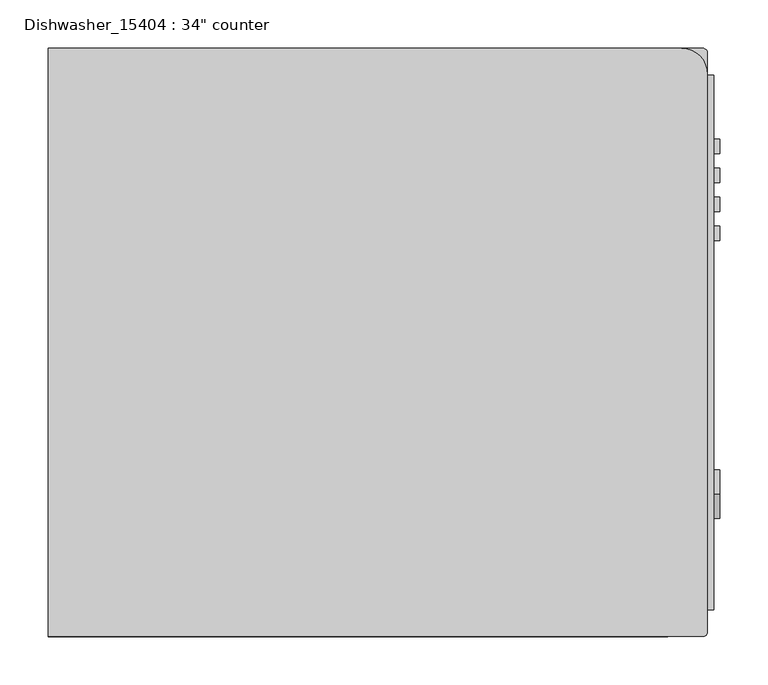
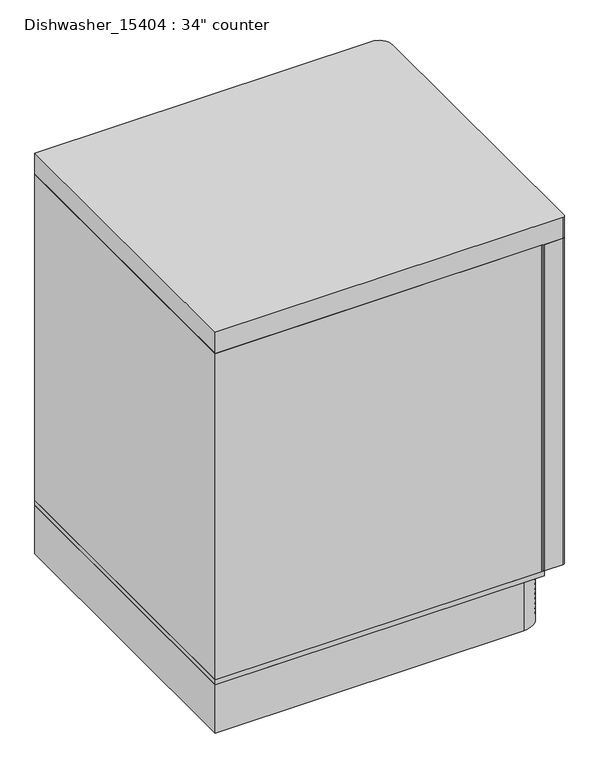
"""IFC4 building model written with IfcOpenShell, lengths in millimetres: proxy geometry."""

from ifc_helpers import new_model, si_unit, point, frame, frame_2d, origin, place, context, project, spatial, polyline, circle_curve, trimmed, segment, composite_curve, outline, extrude, source, transform, mapped, element, save
from ifc_brep_helpers import plane_surface, cylinder_surface, advanced_brep


def proxy_e1c3c540(model_context):
    return source(origin(), model_context, "Body", "SolidModel", [
        extrude(outline(composite_curve([segment(trimmed(circle_curve(frame_2d((147.53066, 741.5840355)), 25.0), [point((147.53066, 716.5840355))], [point((147.53066, 766.5840355))], False, "CARTESIAN"), True, "CONTINUOUS"), segment(trimmed(circle_curve(frame_2d((147.53066, 741.5840355)), 25.0), [point((147.53066, 766.5840355))], [point((147.53066, 716.5840355))], False, "CARTESIAN"), True, "CONTINUOUS")], self_intersect=False)), frame((688.975, 0.0, 0.0), z_axis=(1.0, 0.0, 0.0), x_axis=(0.0, 1.0, 0.0)), (0.0, 0.0, 1.0), 6.35),
        extrude(outline(polyline([(688.975, 410.2108979), (688.975, 425.2108979), (695.325, 425.2108979), (695.325, 410.2108979), (688.975, 410.2108979)])), frame((0.0, 0.0, 745.4030607), z_axis=(0.0, 0.0, 1.0), x_axis=(1.0, 0.0, 0.0)), (0.0, 0.0, 1.0), 15.0),
        extrude(outline(polyline([(688.975, 440.2108979), (688.975, 455.2108979), (695.325, 455.2108979), (695.325, 440.2108979), (688.975, 440.2108979)])), frame((0.0, 0.0, 745.4030607), z_axis=(0.0, 0.0, 1.0), x_axis=(1.0, 0.0, 0.0)), (0.0, 0.0, 1.0), 15.0),
        extrude(outline(polyline([(688.975, 470.2108979), (688.975, 485.2108979), (695.325, 485.2108979), (695.325, 470.2108979), (688.975, 470.2108979)])), frame((0.0, 0.0, 745.4030607), z_axis=(0.0, 0.0, 1.0), x_axis=(1.0, 0.0, 0.0)), (0.0, 0.0, 1.0), 15.0),
        extrude(outline(polyline([(688.975, 500.2108979), (688.975, 515.2108979), (695.325, 515.2108979), (695.325, 500.2108979), (688.975, 500.2108979)])), frame((0.0, 0.0, 745.4030607), z_axis=(0.0, 0.0, 1.0), x_axis=(1.0, 0.0, 0.0)), (0.0, 0.0, 1.0), 15.0),
        extrude(outline(composite_curve([segment(polyline([(512.7209143, 694.5980964), (96.8794309, 694.5980964)]), True, "CONTINUOUS"), segment(trimmed(circle_curve(frame_2d((96.8794309, 729.5980964)), 35.0), [point((96.8794309, 694.5980964))], [point((66.2677412, 712.6297597))], False, "CARTESIAN"), True, "CONTINUOUS"), segment(polyline([(66.2677412, 712.6297597), (27.7608134, 782.0980964), (581.8395319, 782.0980964), (543.3326041, 712.6297597)]), True, "CONTINUOUS"), segment(trimmed(circle_curve(frame_2d((512.7209143, 729.5980964)), 35.0), [point((543.3326041, 712.6297597))], [point((512.7209143, 694.5980964))], False, "CARTESIAN"), True, "CONTINUOUS")], self_intersect=False)), frame((638.175, 0.0, 0.0), z_axis=(1.0, 0.0, 0.0), x_axis=(0.0, 1.0, 0.0)), (0.0, 0.0, 1.0), 50.8),
        extrude(outline(composite_curve([segment(polyline([(0.0, 609.6), (636.35, 609.6)]), True, "CONTINUOUS"), segment(trimmed(circle_curve(frame_2d((636.35, 604.6)), 5.0), [point((636.35, 609.6))], [point((641.35, 604.6))], False, "CARTESIAN"), True, "CONTINUOUS"), segment(polyline([(641.35, 604.6), (641.35, 5.0003453)]), True, "CONTINUOUS"), segment(trimmed(circle_curve(frame_2d((636.35, 5.0003453)), 5.0), [point((641.35, 5.0003453))], [point((636.35, 0.0003453))], False, "CARTESIAN"), True, "CONTINUOUS"), segment(polyline([(636.35, 0.0003453), (0.0, 0.0003453), (0.0, 609.6)]), True, "CONTINUOUS")], self_intersect=False)), frame((0.0, 0.0, 110.0), z_axis=(0.0, 0.0, 1.0), x_axis=(1.0, 0.0, 0.0)), (0.0, 0.0, 1.0), 672.0980964),
        extrude(outline(composite_curve([segment(polyline([(0.0, 609.6), (655.4, 609.6)]), True, "CONTINUOUS"), segment(trimmed(circle_curve(frame_2d((655.4, 582.375)), 27.225), [point((655.4, 609.6))], [point((682.625, 582.375))], False, "CARTESIAN"), True, "CONTINUOUS"), segment(polyline([(682.625, 582.375), (682.625, 5.0)]), True, "CONTINUOUS"), segment(trimmed(circle_curve(frame_2d((677.625, 5.0)), 5.0), [point((682.625, 5.0))], [point((677.625, 0.0))], False, "CARTESIAN"), True, "CONTINUOUS"), segment(polyline([(677.625, 0.0), (0.0, 0.0), (0.0, 609.6)]), True, "CONTINUOUS")], self_intersect=False)), frame((0.0, 0.0, 782.0980964), z_axis=(0.0, 0.0, 1.0), x_axis=(1.0, 0.0, 0.0)), (0.0, 0.0, 1.0), 43.4019036),
        extrude(outline(composite_curve([segment(polyline([(641.35, 609.6), (677.625, 609.6)]), True, "CONTINUOUS"), segment(trimmed(circle_curve(frame_2d((677.625, 604.6)), 5.0), [point((677.625, 609.6))], [point((682.625, 604.6))], False, "CARTESIAN"), True, "CONTINUOUS"), segment(polyline([(682.625, 604.6), (682.625, 5.0)]), True, "CONTINUOUS"), segment(trimmed(circle_curve(frame_2d((677.625, 5.0)), 5.0), [point((682.625, 5.0))], [point((677.625, 0.0))], False, "CARTESIAN"), True, "CONTINUOUS"), segment(polyline([(677.625, 0.0), (641.35, 0.0), (641.35, 609.6)]), True, "CONTINUOUS")], self_intersect=False)), frame((0.0, 0.0, 110.0), z_axis=(0.0, 0.0, 1.0), x_axis=(1.0, 0.0, 0.0)), (0.0, 0.0, 1.0), 672.0980964),
        extrude(outline(polyline([(0.0, 609.6), (641.35, 609.6), (641.35, 0.0), (0.0, 0.0), (0.0, 609.6)])), frame((0.0, 0.0, 100.0), z_axis=(0.0, 0.0, 1.0), x_axis=(1.0, 0.0, 0.0)), (0.0, 0.0, 1.0), 10.0),
        advanced_brep(
        [(0.0, 609.6, 100.0), (0.0, 0.0, 100.0), (601.35, 0.0, 100.0), (641.35, 40.0, 100.0), (641.35, 569.6, 100.0), (601.35, 609.6, 100.0), (0.0, 609.6, 0.0), (601.35, 609.6, 0.0), (641.35, 569.6, 0.0), (641.35, 40.0, 0.0), (601.35, 0.0, 0.0), (0.0, 0.0, 0.0), (641.35, 40.0, 16.3757772), (628.65, 10.7645763, 16.3757772), (628.65, 10.7645763, 21.3757772), (641.35, 40.0, 21.3757772), (641.35, 40.0, 26.2238547), (628.65, 10.7645763, 26.2238547), (628.65, 10.7645763, 31.2238547), (641.35, 40.0, 31.2238547), (641.35, 40.0, 36.2238547), (628.65, 10.7645763, 36.2238547), (628.65, 10.7645763, 41.2238547), (641.35, 40.0, 41.2238547), (641.35, 40.0, 46.2238547), (628.65, 10.7645763, 46.2238547), (628.65, 10.7645763, 51.2238547), (641.35, 40.0, 51.2238547), (641.35, 40.0, 56.2238547), (628.65, 10.7645763, 56.2238547), (628.65, 10.7645763, 61.2238547), (641.35, 40.0, 61.2238547), (641.35, 40.0, 66.2238547), (628.65, 10.7645763, 66.2238547), (628.65, 10.7645763, 71.2238547), (641.35, 40.0, 71.2238547), (641.35, 40.0, 76.2238547), (628.65, 10.7645763, 76.2238547), (628.65, 10.7645763, 81.2238547), (641.35, 40.0, 81.2238547), (641.35, 40.0, 86.2238547), (628.65, 10.7645763, 86.2238547), (628.65, 10.7645763, 91.2238547), (641.35, 40.0, 91.2238547), (641.35, 569.6, 91.2238547), (641.35, 569.6, 16.3757772), (641.35, 569.6, 21.3757772), (641.35, 569.6, 26.2238547), (641.35, 569.6, 31.2238547), (641.35, 569.6, 36.2238547), (641.35, 569.6, 41.2238547), (641.35, 569.6, 46.2238547), (641.35, 569.6, 51.2238547), (641.35, 569.6, 56.2238547), (641.35, 569.6, 61.2238547), (641.35, 569.6, 66.2238547), (641.35, 569.6, 71.2238547), (641.35, 569.6, 76.2238547), (641.35, 569.6, 81.2238547), (641.35, 569.6, 86.2238547), (628.65, 598.8354237, 91.2238547), (628.65, 598.8354237, 86.2238547), (628.65, 598.8354237, 81.2238547), (628.65, 598.8354237, 76.2238547), (628.65, 598.8354237, 71.2238547), (628.65, 598.8354237, 66.2238547), (628.65, 598.8354237, 61.2238547), (628.65, 598.8354237, 56.2238547), (628.65, 598.8354237, 51.2238547), (628.65, 598.8354237, 46.2238547), (628.65, 598.8354237, 41.2238547), (628.65, 598.8354237, 36.2238547), (628.65, 598.8354237, 31.2238547), (628.65, 598.8354237, 26.2238547), (628.65, 598.8354237, 21.3757772), (628.65, 598.8354237, 16.3757772)],
        [
            (0, 1),
            (1, 2),
            (2, 3, circle_curve(frame((601.35, 40.0, 100.0), z_axis=(0.0, 0.0, 1.0), x_axis=(1.0, 0.0, 0.0)), 40.0)),
            (3, 4),
            (4, 5, circle_curve(frame((601.35, 569.6, 100.0), z_axis=(0.0, 0.0, 1.0), x_axis=(1.0, 0.0, 0.0)), 40.0)),
            (5, 0),
            (6, 7),
            (7, 8, circle_curve(frame((601.35, 569.6, 0.0), z_axis=(0.0, 0.0, -1.0), x_axis=(1.0, 0.0, 0.0)), 40.0)),
            (8, 9),
            (9, 10, circle_curve(frame((601.35, 40.0, 0.0), z_axis=(0.0, 0.0, -1.0), x_axis=(1.0, 0.0, 0.0)), 40.0)),
            (10, 11),
            (11, 6),
            (0, 6),
            (11, 1),
            (10, 2),
            (9, 12),
            (12, 13, circle_curve(frame((601.35, 40.0, 16.3757772), z_axis=(0.0, 0.0, -1.0), x_axis=(1.0, 0.0, 0.0)), 40.0)),
            (13, 14),
            (14, 15, circle_curve(frame((601.35, 40.0, 21.3757772), z_axis=(0.0, 0.0, 1.0), x_axis=(1.0, 0.0, 0.0)), 40.0)),
            (15, 16),
            (16, 17, circle_curve(frame((601.35, 40.0, 26.2238547), z_axis=(0.0, 0.0, -1.0), x_axis=(1.0, 0.0, 0.0)), 40.0)),
            (17, 18),
            (18, 19, circle_curve(frame((601.35, 40.0, 31.2238547), z_axis=(0.0, 0.0, 1.0), x_axis=(1.0, 0.0, 0.0)), 40.0)),
            (19, 20),
            (20, 21, circle_curve(frame((601.35, 40.0, 36.2238547), z_axis=(0.0, 0.0, -1.0), x_axis=(1.0, 0.0, 0.0)), 40.0)),
            (21, 22),
            (22, 23, circle_curve(frame((601.35, 40.0, 41.2238547), z_axis=(0.0, 0.0, 1.0), x_axis=(1.0, 0.0, 0.0)), 40.0)),
            (23, 24),
            (24, 25, circle_curve(frame((601.35, 40.0, 46.2238547), z_axis=(0.0, 0.0, -1.0), x_axis=(1.0, 0.0, 0.0)), 40.0)),
            (25, 26),
            (26, 27, circle_curve(frame((601.35, 40.0, 51.2238547), z_axis=(0.0, 0.0, 1.0), x_axis=(1.0, 0.0, 0.0)), 40.0)),
            (27, 28),
            (28, 29, circle_curve(frame((601.35, 40.0, 56.2238547), z_axis=(0.0, 0.0, -1.0), x_axis=(1.0, 0.0, 0.0)), 40.0)),
            (29, 30),
            (30, 31, circle_curve(frame((601.35, 40.0, 61.2238547), z_axis=(0.0, 0.0, 1.0), x_axis=(1.0, 0.0, 0.0)), 40.0)),
            (31, 32),
            (32, 33, circle_curve(frame((601.35, 40.0, 66.2238547), z_axis=(0.0, 0.0, -1.0), x_axis=(1.0, 0.0, 0.0)), 40.0)),
            (33, 34),
            (34, 35, circle_curve(frame((601.35, 40.0, 71.2238547), z_axis=(0.0, 0.0, 1.0), x_axis=(1.0, 0.0, 0.0)), 40.0)),
            (35, 36),
            (36, 37, circle_curve(frame((601.35, 40.0, 76.2238547), z_axis=(0.0, 0.0, -1.0), x_axis=(1.0, 0.0, 0.0)), 40.0)),
            (37, 38),
            (38, 39, circle_curve(frame((601.35, 40.0, 81.2238547), z_axis=(0.0, 0.0, 1.0), x_axis=(1.0, 0.0, 0.0)), 40.0)),
            (39, 40),
            (40, 41, circle_curve(frame((601.35, 40.0, 86.2238547), z_axis=(0.0, 0.0, -1.0), x_axis=(1.0, 0.0, 0.0)), 40.0)),
            (41, 42),
            (42, 43, circle_curve(frame((601.35, 40.0, 91.2238547), z_axis=(0.0, 0.0, 1.0), x_axis=(1.0, 0.0, 0.0)), 40.0)),
            (43, 3),
            (43, 44),
            (44, 4),
            (8, 45),
            (45, 12),
            (15, 46),
            (46, 47),
            (47, 16),
            (19, 48),
            (48, 49),
            (49, 20),
            (23, 50),
            (50, 51),
            (51, 24),
            (27, 52),
            (52, 53),
            (53, 28),
            (31, 54),
            (54, 55),
            (55, 32),
            (35, 56),
            (56, 57),
            (57, 36),
            (39, 58),
            (58, 59),
            (59, 40),
            (44, 60, circle_curve(frame((601.35, 569.6, 91.2238547), z_axis=(0.0, 0.0, 1.0), x_axis=(1.0, 0.0, 0.0)), 40.0)),
            (60, 61),
            (61, 59, circle_curve(frame((601.35, 569.6, 86.2238547), z_axis=(0.0, 0.0, -1.0), x_axis=(1.0, 0.0, 0.0)), 40.0)),
            (58, 62, circle_curve(frame((601.35, 569.6, 81.2238547), z_axis=(0.0, 0.0, 1.0), x_axis=(1.0, 0.0, 0.0)), 40.0)),
            (62, 63),
            (63, 57, circle_curve(frame((601.35, 569.6, 76.2238547), z_axis=(0.0, 0.0, -1.0), x_axis=(1.0, 0.0, 0.0)), 40.0)),
            (56, 64, circle_curve(frame((601.35, 569.6, 71.2238547), z_axis=(0.0, 0.0, 1.0), x_axis=(1.0, 0.0, 0.0)), 40.0)),
            (64, 65),
            (65, 55, circle_curve(frame((601.35, 569.6, 66.2238547), z_axis=(0.0, 0.0, -1.0), x_axis=(1.0, 0.0, 0.0)), 40.0)),
            (54, 66, circle_curve(frame((601.35, 569.6, 61.2238547), z_axis=(0.0, 0.0, 1.0), x_axis=(1.0, 0.0, 0.0)), 40.0)),
            (66, 67),
            (67, 53, circle_curve(frame((601.35, 569.6, 56.2238547), z_axis=(0.0, 0.0, -1.0), x_axis=(1.0, 0.0, 0.0)), 40.0)),
            (52, 68, circle_curve(frame((601.35, 569.6, 51.2238547), z_axis=(0.0, 0.0, 1.0), x_axis=(1.0, 0.0, 0.0)), 40.0)),
            (68, 69),
            (69, 51, circle_curve(frame((601.35, 569.6, 46.2238547), z_axis=(0.0, 0.0, -1.0), x_axis=(1.0, 0.0, 0.0)), 40.0)),
            (50, 70, circle_curve(frame((601.35, 569.6, 41.2238547), z_axis=(0.0, 0.0, 1.0), x_axis=(1.0, 0.0, 0.0)), 40.0)),
            (70, 71),
            (71, 49, circle_curve(frame((601.35, 569.6, 36.2238547), z_axis=(0.0, 0.0, -1.0), x_axis=(1.0, 0.0, 0.0)), 40.0)),
            (48, 72, circle_curve(frame((601.35, 569.6, 31.2238547), z_axis=(0.0, 0.0, 1.0), x_axis=(1.0, 0.0, 0.0)), 40.0)),
            (72, 73),
            (73, 47, circle_curve(frame((601.35, 569.6, 26.2238547), z_axis=(0.0, 0.0, -1.0), x_axis=(1.0, 0.0, 0.0)), 40.0)),
            (46, 74, circle_curve(frame((601.35, 569.6, 21.3757772), z_axis=(0.0, 0.0, 1.0), x_axis=(1.0, 0.0, 0.0)), 40.0)),
            (74, 75),
            (75, 45, circle_curve(frame((601.35, 569.6, 16.3757772), z_axis=(0.0, 0.0, -1.0), x_axis=(1.0, 0.0, 0.0)), 40.0)),
            (7, 5),
            (60, 42),
            (41, 61),
            (62, 38),
            (37, 63),
            (64, 34),
            (33, 65),
            (66, 30),
            (29, 67),
            (68, 26),
            (25, 69),
            (70, 22),
            (21, 71),
            (72, 18),
            (17, 73),
            (74, 14),
            (13, 75),
        ],
        [
            plane_surface(frame((0.0, 0.0, 100.0), z_axis=(0.0, 0.0, 1.0), x_axis=(0.0, -1.0, 0.0))),
            plane_surface(frame((0.0, 0.0, 0.0), z_axis=(0.0, 0.0, -1.0), x_axis=(0.0, 1.0, 0.0))),
            plane_surface(frame((0.0, 609.6, 100.0), z_axis=(-1.0, 0.0, 0.0), x_axis=(0.0, 0.0, -1.0))),
            plane_surface(frame((0.0, 0.0, 100.0), z_axis=(0.0, -1.0, 0.0), x_axis=(0.0, 0.0, -1.0))),
            cylinder_surface(frame((601.35, 40.0, 0.0), z_axis=(0.0, 0.0, 1.0), x_axis=(1.0, 0.0, 0.0)), 40.0),
            plane_surface(frame((641.35, 40.0, 100.0), z_axis=(1.0, 0.0, 0.0), x_axis=(0.0, 0.0, -1.0))),
            cylinder_surface(frame((601.35, 569.6, 0.0), z_axis=(0.0, 0.0, 1.0), x_axis=(1.0, 0.0, 0.0)), 40.0),
            plane_surface(frame((601.35, 609.6, 100.0), z_axis=(0.0, 1.0, 0.0), x_axis=(0.0, 0.0, -1.0))),
            plane_surface(frame((628.65, 0.0, 91.2238547), z_axis=(1.0, 0.0, 0.0), x_axis=(0.0, 1.0, 0.0))),
            plane_surface(frame((666.75, 609.6, 91.2238547), z_axis=(0.0, 0.0, -1.0), x_axis=(-1.0, 0.0, 0.0))),
            plane_surface(frame((666.75, 0.0, 86.2238547), z_axis=(0.0, 0.0, 1.0), x_axis=(-1.0, 0.0, 0.0))),
            plane_surface(frame((666.75, 609.6, 81.2238547), z_axis=(0.0, 0.0, -1.0), x_axis=(-1.0, 0.0, 0.0))),
            plane_surface(frame((666.75, 0.0, 76.2238547), z_axis=(0.0, 0.0, 1.0), x_axis=(-1.0, 0.0, 0.0))),
            plane_surface(frame((666.75, 609.6, 71.2238547), z_axis=(0.0, 0.0, -1.0), x_axis=(-1.0, 0.0, 0.0))),
            plane_surface(frame((666.75, 0.0, 66.2238547), z_axis=(0.0, 0.0, 1.0), x_axis=(-1.0, 0.0, 0.0))),
            plane_surface(frame((666.75, 609.6, 61.2238547), z_axis=(0.0, 0.0, -1.0), x_axis=(-1.0, 0.0, 0.0))),
            plane_surface(frame((666.75, 0.0, 56.2238547), z_axis=(0.0, 0.0, 1.0), x_axis=(-1.0, 0.0, 0.0))),
            plane_surface(frame((666.75, 609.6, 51.2238547), z_axis=(0.0, 0.0, -1.0), x_axis=(-1.0, 0.0, 0.0))),
            plane_surface(frame((666.75, 0.0, 46.2238547), z_axis=(0.0, 0.0, 1.0), x_axis=(-1.0, 0.0, 0.0))),
            plane_surface(frame((666.75, 609.6, 41.2238547), z_axis=(0.0, 0.0, -1.0), x_axis=(-1.0, 0.0, 0.0))),
            plane_surface(frame((666.75, 0.0, 36.2238547), z_axis=(0.0, 0.0, 1.0), x_axis=(-1.0, 0.0, 0.0))),
            plane_surface(frame((666.75, 609.6, 31.2238547), z_axis=(0.0, 0.0, -1.0), x_axis=(-1.0, 0.0, 0.0))),
            plane_surface(frame((666.75, 0.0, 26.2238547), z_axis=(0.0, 0.0, 1.0), x_axis=(-1.0, 0.0, 0.0))),
            plane_surface(frame((666.75, 609.6, 21.3757772), z_axis=(0.0, 0.0, -1.0), x_axis=(-1.0, 0.0, 0.0))),
            plane_surface(frame((666.75, 0.0, 16.3757772), z_axis=(0.0, 0.0, 1.0), x_axis=(-1.0, 0.0, 0.0))),
        ],
        [
            (0, [[1, 2, 3, 4, 5, 6]]),
            (1, [[7, 8, 9, 10, 11, 12]]),
            (2, [[-1, 13, -12, 14]]),
            (3, [[-2, -14, -11, 15]]),
            (4, [[-3, -15, -10, 16, 17, 18, 19, 20, 21, 22, 23, 24, 25, 26, 27, 28, 29, 30, 31, 32, 33, 34, 35, 36, 37, 38, 39, 40, 41, 42, 43, 44, 45, 46, 47, 48]]),
            (5, [[-4, -48, 49, 50]]),
            (5, [[-9, 51, 52, -16]]),
            (5, [[-20, 53, 54, 55]]),
            (5, [[-24, 56, 57, 58]]),
            (5, [[-28, 59, 60, 61]]),
            (5, [[-32, 62, 63, 64]]),
            (5, [[-36, 65, 66, 67]]),
            (5, [[-40, 68, 69, 70]]),
            (5, [[-44, 71, 72, 73]]),
            (6, [[-5, -50, 74, 75, 76, -72, 77, 78, 79, -69, 80, 81, 82, -66, 83, 84, 85, -63, 86, 87, 88, -60, 89, 90, 91, -57, 92, 93, 94, -54, 95, 96, 97, -51, -8, 98]]),
            (7, [[-6, -98, -7, -13]]),
            (8, [[99, -46, 100, -75]]),
            (8, [[101, -42, 102, -78]]),
            (8, [[103, -38, 104, -81]]),
            (8, [[105, -34, 106, -84]]),
            (8, [[107, -30, 108, -87]]),
            (8, [[109, -26, 110, -90]]),
            (8, [[111, -22, 112, -93]]),
            (8, [[113, -18, 114, -96]]),
            (9, [[-99, -74, -49, -47]]),
            (10, [[-100, -45, -73, -76]]),
            (11, [[-101, -77, -71, -43]]),
            (12, [[-102, -41, -70, -79]]),
            (13, [[-103, -80, -68, -39]]),
            (14, [[-104, -37, -67, -82]]),
            (15, [[-105, -83, -65, -35]]),
            (16, [[-106, -33, -64, -85]]),
            (17, [[-107, -86, -62, -31]]),
            (18, [[-108, -29, -61, -88]]),
            (19, [[-109, -89, -59, -27]]),
            (20, [[-110, -25, -58, -91]]),
            (21, [[-111, -92, -56, -23]]),
            (22, [[-112, -21, -55, -94]]),
            (23, [[-113, -95, -53, -19]]),
            (24, [[-114, -17, -52, -97]]),
        ],
    ),
    ])


if __name__ == "__main__":
    model = new_model("IFC4")
    model_context = context("Model", 3, world=origin())
    ifc_project = project(units=[si_unit("LENGTHUNIT", "METRE", prefix="MILLI")], contexts=[model_context])
    site = spatial("IfcSite", under=ifc_project)
    building = spatial("IfcBuilding", under=site)
    placement = place(None, origin())
    proxy_shape = proxy_e1c3c540(model_context)
    element("IfcBuildingElementProxy", 1, Name="Dishwasher_15404 : 34\" counter", ObjectType="Dishwasher_15404 : 34\" counter", at=placement, inside=building, context=model_context, shape_type="MappedRepresentation", body=[
        mapped(proxy_shape, transform((0.0, 0.0, 0.0), x_axis=(1.0, 0.0, 0.0), y_axis=(0.0, 1.0, 0.0), z_axis=(0.0, 0.0, 1.0))),
    ])
    save(model, "model.ifc")

# Revit data of these elements
# Type "Dishwasher_15404 : 34\" counter"
#   Width = 2' - 0"
#   Height = 2' - 8 1/2"
#   Depth = 2' - 0"
